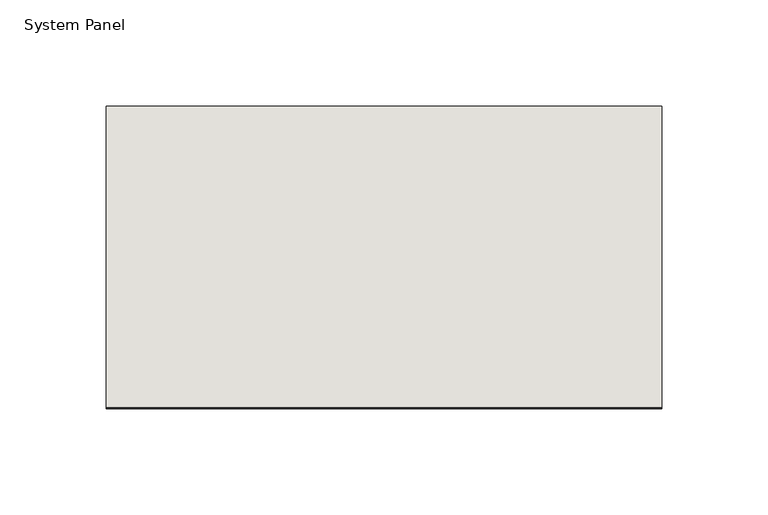
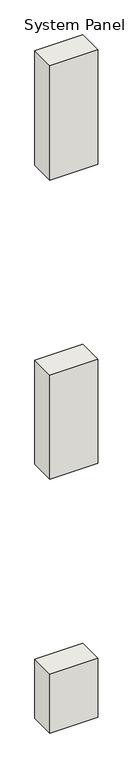
"""IFC4 building model written with IfcOpenShell, lengths in millimetres: wall geometry, System Panel : NLRS_21_CWP_hsb-vulling minerale wol 142 _gen_rsf."""

from ifc_helpers import new_model, si_unit, frame, origin, origin_with_axes, place, context, project, spatial, polyline, outline, extrude, source, transform, mapped, element, save


def system_panel_51be6294(model_context):
    return source(origin(), model_context, "Body", "SweptSolid", [
        extrude(outline(polyline([(131.0, -71.0), (-131.0, -71.0), (-131.0, 71.0), (131.0, 71.0), (131.0, -71.0)])), origin_with_axes(), (0.0, 0.0, 1.0), 339.0),
        extrude(outline(polyline([(131.0, -71.0), (-131.0, -71.0), (-131.0, 71.0), (131.0, 71.0), (131.0, -71.0)])), frame((0.0, 0.0, 1465.0), z_axis=(0.0, 0.0, 1.0), x_axis=(1.0, 0.0, 0.0)), (0.0, 0.0, 1.0), 599.0),
        extrude(outline(polyline([(131.0, -71.0), (-131.0, -71.0), (-131.0, 71.0), (131.0, 71.0), (131.0, -71.0)])), frame((0.0, 0.0, 3190.0), z_axis=(0.0, 0.0, 1.0), x_axis=(1.0, 0.0, 0.0)), (0.0, 0.0, 1.0), 659.0),
    ])


if __name__ == "__main__":
    model = new_model("IFC4")
    model_context = context("Model", 3, world=origin())
    ifc_project = project(units=[si_unit("LENGTHUNIT", "METRE", prefix="MILLI")], contexts=[model_context])
    site = spatial("IfcSite", under=ifc_project)
    building = spatial("IfcBuilding", under=site)
    placement = place(None, origin())
    system_panel_shape = system_panel_51be6294(model_context)
    element("IfcWall", 1, ObjectType="System Panel : NLRS_21_CWP_hsb-vulling minerale wol 142 _gen_rsf", at=placement, inside=building, context=model_context, shape_type="MappedRepresentation", body=[
        mapped(system_panel_shape, transform((0.0, 0.0, 0.0), x_axis=(1.0, 0.0, 0.0), y_axis=(0.0, 1.0, 0.0), z_axis=(0.0, 0.0, 1.0))),
    ])
    save(model, "model.ifc")

# Revit data of these elements
# Type "System Panel : NLRS_21_CWP_hsb-vulling minerale wol 142 _gen_rsf"
#   Type IfcGUID = "07M7mRoiH1CR8m_RSKIwpC"
#   Assembly Code = "21.23"
#   IfcExportAs = "IfcWall"
# Element 1 (IfcWall, "System Panel : NLRS_21_CWP_hsb-vulling minerale wol 142 _gen_rsf")
#   Materials on its faces: "NLRS_m1_isolatie minerale wol_gen_rsf"
# Materials
#   "NLRS_m1_isolatie minerale wol_gen_rsf": class "M - Anorganische materialen", colour RGB 200 200 140, transparency 0, Keynote = "m1", Manufacturer = "Revit Standards Foundation", URL = "www.revitstandards.org", Description = "isolatie minerale wol", Cost = 0
